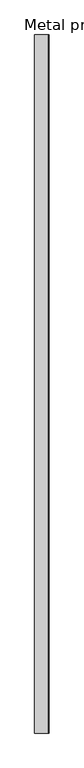
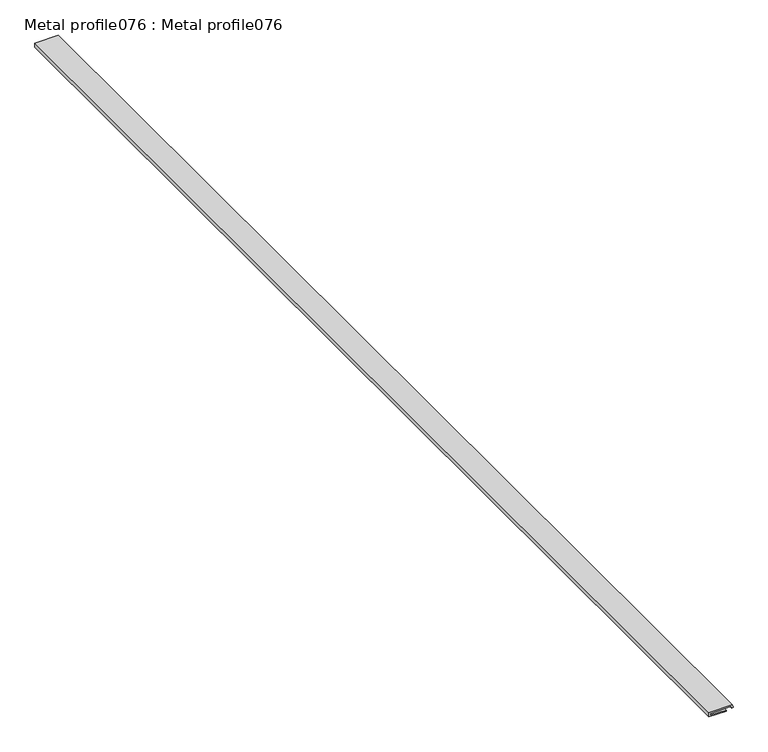
"""IFC4 building model written with IfcOpenShell, lengths in millimetres: proxy geometry, Metal profile076 : Metal profile076."""

from ifc_helpers import new_model, si_unit, frame, origin, place, context, project, spatial, polyline, outline, extrude, source, transform, mapped, element, save


def metal_profile076_metal_profile076_a0c68145(model_context):
    return source(origin(), model_context, "Body", "SweptSolid", [
        extrude(outline(polyline([(40172.6132812, -9789.3759766), (40172.6132812, -9816.6435547), (40175.9203326, -9816.6435547), (40176.4624429, -9780.4202469), (40172.8172405, -9779.2476693), (40173.4296875, -9777.34375), (40178.484375, -9778.9697266), (40177.890625, -9818.6435547), (40170.6132812, -9818.6435547), (40170.6132812, -9789.3759766), (40172.6132812, -9789.3759766)])), frame((0.0, 7982.1531721, 0.0), z_axis=(0.0, 1.0, 0.0), x_axis=(0.0, 0.0, 1.0)), (0.0, 0.0, 1.0), 2000.0),
    ])


if __name__ == "__main__":
    model = new_model("IFC4")
    model_context = context("Model", 3, world=origin())
    ifc_project = project(units=[si_unit("LENGTHUNIT", "METRE", prefix="MILLI")], contexts=[model_context])
    site = spatial("IfcSite", under=ifc_project)
    building = spatial("IfcBuilding", under=site)
    placement = place(None, origin())
    metal_profile076_metal_profile076_shape = metal_profile076_metal_profile076_a0c68145(model_context)
    element("IfcBuildingElementProxy", 1, Name="Metal profile076 : Metal profile076", ObjectType="Metal profile076 : Metal profile076", at=placement, inside=building, context=model_context, shape_type="MappedRepresentation", body=[
        mapped(metal_profile076_metal_profile076_shape, transform((0.0, 0.0, 0.0), x_axis=(1.0, 0.0, 0.0), y_axis=(0.0, 1.0, 0.0), z_axis=(0.0, 0.0, 1.0))),
    ])
    save(model, "model.ifc")

# Revit data of these elements
# Type "Metal profile076 : Metal profile076"
#   NameOverride = "Metal profile076"
# Element 1 (IfcBuildingElementProxy, "Metal profile076 : Metal profile076")
#   Materials on its faces: "ANGLE TRIM"
# Materials
#   "ANGLE TRIM": class "Unassigned", colour RGB 250 255 0, transparency 0
